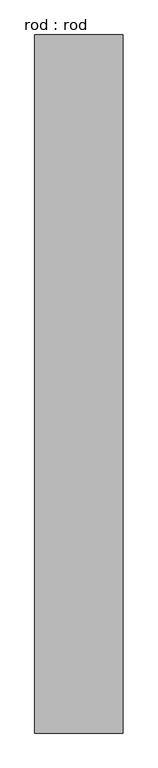
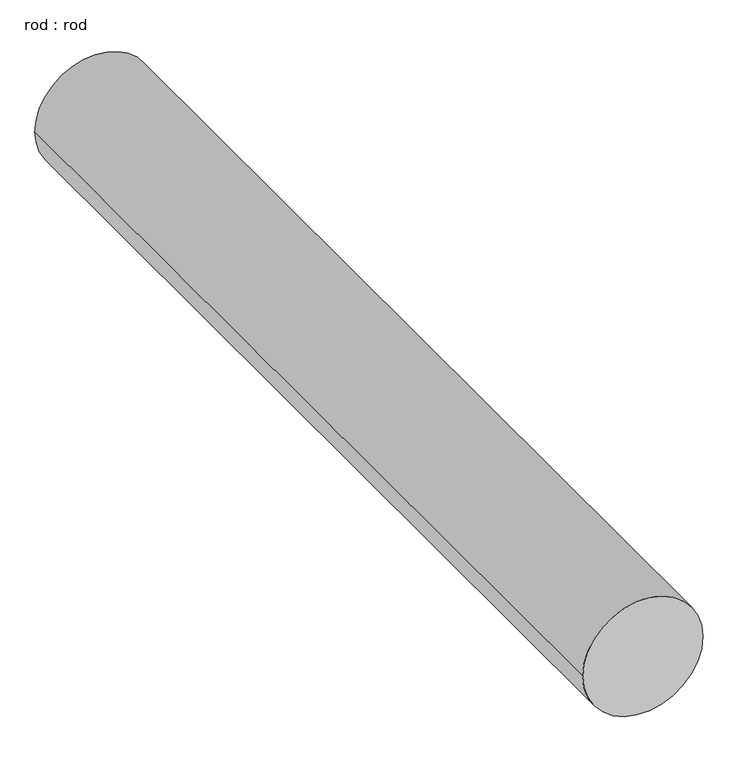
"""IFC4 building model written with IfcOpenShell, lengths in millimetres: proxy geometry, rod : rod."""

from ifc_helpers import new_model, si_unit, point, frame, frame_2d, origin, place, context, project, spatial, circle_curve, trimmed, segment, composite_curve, outline, extrude, source, transform, mapped, element, save


def rod_rod_140f7cf2(model_context):
    return source(origin(), model_context, "Body", "SweptSolid", [
        extrude(outline(composite_curve([segment(trimmed(circle_curve(frame_2d((0.0108462, 0.0)), 200.0), [point((0.0108462, 200.0))], [point((0.0108462, -200.0))], False, "CARTESIAN"), True, "CONTINUOUS"), segment(trimmed(circle_curve(frame_2d((0.0108462, 0.0)), 200.0), [point((0.0108462, -200.0))], [point((0.0108462, 200.0))], False, "CARTESIAN"), True, "CONTINUOUS")], self_intersect=False)), frame((0.0, 2512.7286153, 0.0), z_axis=(0.0, 1.0, 0.0), x_axis=(0.0, 0.0, 1.0)), (0.0, 0.0, 1.0), 3160.0),
    ])


if __name__ == "__main__":
    model = new_model("IFC4")
    model_context = context("Model", 3, world=origin())
    ifc_project = project(units=[si_unit("LENGTHUNIT", "METRE", prefix="MILLI")], contexts=[model_context])
    site = spatial("IfcSite", under=ifc_project)
    building = spatial("IfcBuilding", under=site)
    placement = place(None, origin())
    rod_rod_shape = rod_rod_140f7cf2(model_context)
    element("IfcBuildingElementProxy", 1, Name="rod : rod", ObjectType="rod : rod", at=placement, inside=building, context=model_context, shape_type="MappedRepresentation", body=[
        mapped(rod_rod_shape, transform((0.0, 0.0, 0.0), x_axis=(1.0, 0.0, 0.0), y_axis=(0.0, 1.0, 0.0), z_axis=(0.0, 0.0, 1.0))),
    ])
    save(model, "model.ifc")

# Revit data of these elements
# Type "rod : rod"
#   Default Elevation = 0
